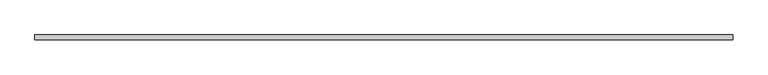
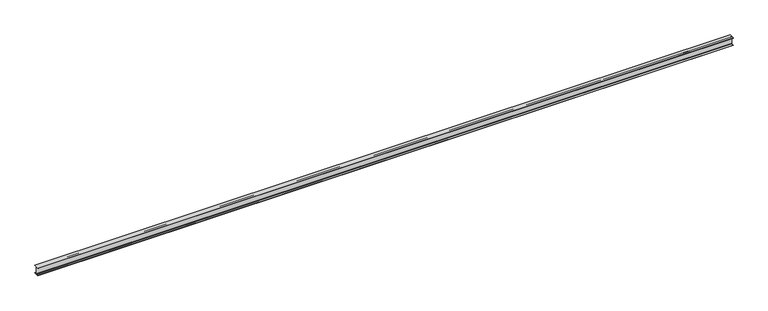
"""IFC4 building model written with IfcOpenShell, lengths in millimetres: beam geometry, Steel Framing_H_KS : H_SB_AR_S02_H-488x300x11x18_CRG1."""

from ifc_helpers import new_model, si_unit, point, frame, frame_2d, origin, place, context, project, spatial, polyline, circle_curve, trimmed, segment, composite_curve, outline, extrude, source, transform, mapped, element, save


def beam_632170ba(model_context):
    return source(origin(), model_context, "Body", "SweptSolid", [
        extrude(outline(composite_curve([segment(polyline([(150.0, -226.0), (150.0, -244.0), (-150.0, -244.0), (-150.0, -226.0), (-31.5, -226.0)]), True, "CONTINUOUS"), segment(trimmed(circle_curve(frame_2d((-31.5, -200.0)), 26.0), [point((-31.5, -226.0))], [point((-5.5, -200.0))], True, "CARTESIAN"), True, "CONTINUOUS"), segment(polyline([(-5.5, -200.0), (-5.5, 200.0)]), True, "CONTINUOUS"), segment(trimmed(circle_curve(frame_2d((-31.5, 200.0)), 26.0), [point((-5.5, 200.0))], [point((-31.5, 226.0))], True, "CARTESIAN"), True, "CONTINUOUS"), segment(polyline([(-31.5, 226.0), (-150.0, 226.0), (-150.0, 244.0), (150.0, 244.0), (150.0, 226.0), (31.5, 226.0)]), True, "CONTINUOUS"), segment(trimmed(circle_curve(frame_2d((31.5, 200.0)), 26.0), [point((31.5, 226.0))], [point((5.5, 200.0))], True, "CARTESIAN"), True, "CONTINUOUS"), segment(polyline([(5.5, 200.0), (5.5, -200.0)]), True, "CONTINUOUS"), segment(trimmed(circle_curve(frame_2d((31.5, -200.0)), 26.0), [point((5.5, -200.0))], [point((31.5, -226.0))], True, "CARTESIAN"), True, "CONTINUOUS"), segment(polyline([(31.5, -226.0), (150.0, -226.0)]), True, "CONTINUOUS")], self_intersect=False)), frame((-20987.2, 0.0, 0.0), z_axis=(1.0, 0.0, 0.0), x_axis=(0.0, 1.0, 0.0)), (0.0, 0.0, 1.0), 41974.4),
    ])


if __name__ == "__main__":
    model = new_model("IFC4")
    model_context = context("Model", 3, world=origin())
    ifc_project = project(units=[si_unit("LENGTHUNIT", "METRE", prefix="MILLI")], contexts=[model_context])
    site = spatial("IfcSite", under=ifc_project)
    building = spatial("IfcBuilding", under=site)
    placement = place(None, origin())
    beam_shape = beam_632170ba(model_context)
    element("IfcBeam", 1, ObjectType="Steel Framing_H_KS : H_SB_AR_S02_H-488x300x11x18_CRG1", at=placement, inside=building, context=model_context, shape_type="MappedRepresentation", body=[
        mapped(beam_shape, transform((0.0, 0.0, 0.0), x_axis=(1.0, 0.0, 0.0), y_axis=(0.0, 1.0, 0.0), z_axis=(0.0, 0.0, 1.0))),
    ])
    save(model, "model.ifc")

# Revit data of these elements
# Type "Steel Framing_H_KS : H_SB_AR_S02_H-488x300x11x18_CRG1"
#   Type Comments = "MAIN"
#   Type Mark = "CRG1"
#   H_SectionID = "H-488x300x11x18"
#   H_Ratio for Additional Steel Plate = 0.2
#   Width = 30.0 cm
#   Web Thickness = 1.1 cm
#   Web Fillet = 2.6 cm
#   Warping Constant = 4470000.0 cm⁶
#   Torsional Moment of Inertia = 137.492 cm⁴
#   Section Area = 163.5 cm²
#   Plastic Modulus weak axis = 830.0 cm³
#   Plastic Modulus strong axis = 3230.0 cm³
#   Perimeter = 2.11 m²/m
#   Nominal Weight = 128.00 kgf/m
#   Moment of Inertia weak axis = 8110.00 cm⁴
#   Moment of Inertia strong axis = 71000.00 cm⁴
#   Height = 48.8 cm
#   Flange Thickness = 1.8 cm
#   Elastic Modulus weak axis = 541.0 cm³
#   Elastic Modulus strong axis = 2910.0 cm³
#   Centroid Vertical = 24.4 cm
#   Centroid Horizontal = 15.0 cm
#   Bolt Spacing = 8.89 cm
#   Length [instance default] = 1500 mm
#   Structural Material [instance default] = Steel, 45-345
#   Section Name Key = ""
#   Assembly Code = ""
# Element 1 (IfcBeam, "Steel Framing_H_KS : H_SB_AR_S02_H-488x300x11x18_CRG1")
#   Materials on its faces: "Steel, 45-345"
# Materials
#   "Steel, 45-345": class "Metal", colour RGB 189 187 185, transparency 0, Description = "Steel 345 MPa", Cost = 0
